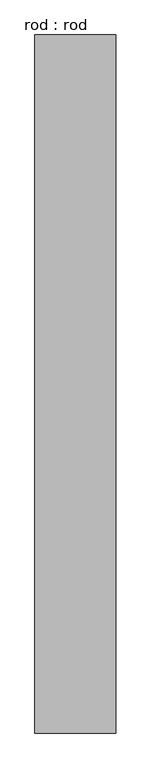
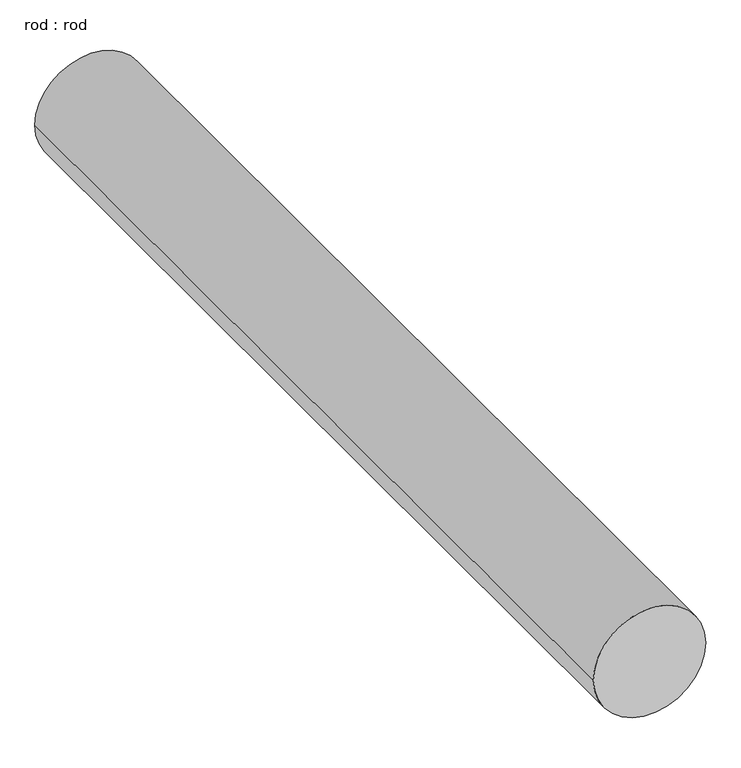
"""IFC4 building model written with IfcOpenShell, lengths in millimetres: proxy geometry, rod : rod."""

from ifc_helpers import new_model, si_unit, point, frame, frame_2d, origin, place, context, project, spatial, circle_curve, trimmed, segment, composite_curve, outline, extrude, source, transform, mapped, element, save


def rod_rod_2daf11ef(model_context):
    return source(origin(), model_context, "Body", "SweptSolid", [
        extrude(outline(composite_curve([segment(trimmed(circle_curve(frame_2d((0.0108462, 0.0)), 200.0), [point((0.0108462, 200.0))], [point((0.0108462, -200.0))], False, "CARTESIAN"), True, "CONTINUOUS"), segment(trimmed(circle_curve(frame_2d((0.0108462, 0.0)), 200.0), [point((0.0108462, -200.0))], [point((0.0108462, 200.0))], False, "CARTESIAN"), True, "CONTINUOUS")], self_intersect=False)), frame((0.0, 2367.7286153, 0.0), z_axis=(0.0, 1.0, 0.0), x_axis=(0.0, 0.0, 1.0)), (0.0, 0.0, 1.0), 3450.0),
    ])


if __name__ == "__main__":
    model = new_model("IFC4")
    model_context = context("Model", 3, world=origin())
    ifc_project = project(units=[si_unit("LENGTHUNIT", "METRE", prefix="MILLI")], contexts=[model_context])
    site = spatial("IfcSite", under=ifc_project)
    building = spatial("IfcBuilding", under=site)
    placement = place(None, origin())
    rod_rod_shape = rod_rod_2daf11ef(model_context)
    element("IfcBuildingElementProxy", 1, Name="rod : rod", ObjectType="rod : rod", at=placement, inside=building, context=model_context, shape_type="MappedRepresentation", body=[
        mapped(rod_rod_shape, transform((0.0, 0.0, 0.0), x_axis=(1.0, 0.0, 0.0), y_axis=(0.0, 1.0, 0.0), z_axis=(0.0, 0.0, 1.0))),
    ])
    save(model, "model.ifc")

# Revit data of these elements
# Type "rod : rod"
#   Default Elevation = 0
